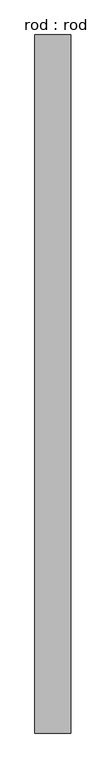
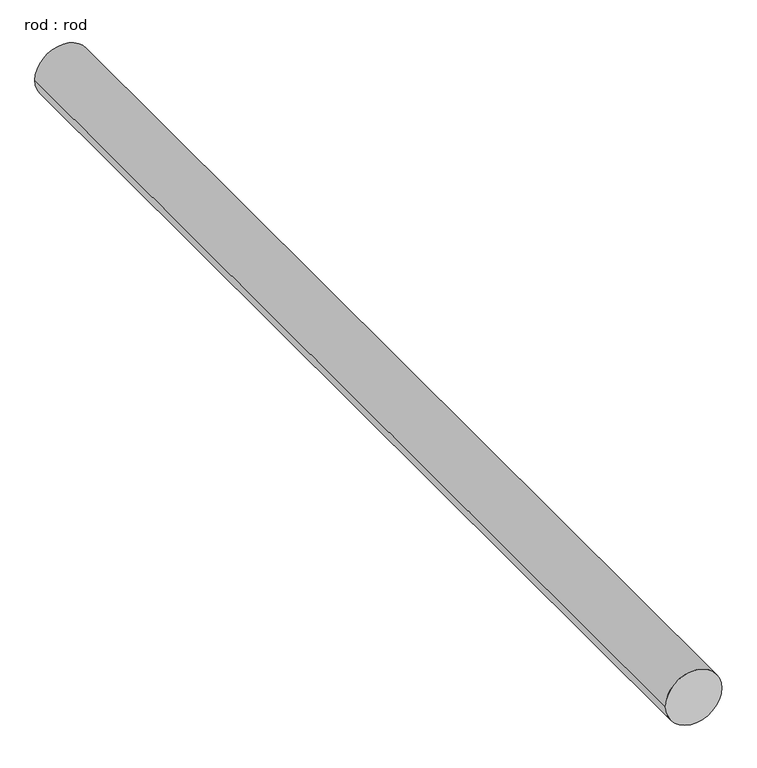
"""IFC4 building model written with IfcOpenShell, lengths in millimetres: proxy geometry, rod : rod."""

from ifc_helpers import new_model, si_unit, point, frame, frame_2d, origin, place, context, project, spatial, circle_curve, trimmed, segment, composite_curve, outline, extrude, source, transform, mapped, element, save


def rod_rod_ac49b040(model_context):
    return source(origin(), model_context, "Body", "SweptSolid", [
        extrude(outline(composite_curve([segment(trimmed(circle_curve(frame_2d((0.0108462, 0.0)), 200.0), [point((0.0108462, 200.0))], [point((0.0108462, -200.0))], False, "CARTESIAN"), True, "CONTINUOUS"), segment(trimmed(circle_curve(frame_2d((0.0108462, 0.0)), 200.0), [point((0.0108462, -200.0))], [point((0.0108462, 200.0))], False, "CARTESIAN"), True, "CONTINUOUS")], self_intersect=False)), frame((0.0, 207.8192318, 0.0), z_axis=(0.0, 1.0, 0.0), x_axis=(0.0, 0.0, 1.0)), (0.0, 0.0, 1.0), 7769.8187671),
    ])


if __name__ == "__main__":
    model = new_model("IFC4")
    model_context = context("Model", 3, world=origin())
    ifc_project = project(units=[si_unit("LENGTHUNIT", "METRE", prefix="MILLI")], contexts=[model_context])
    site = spatial("IfcSite", under=ifc_project)
    building = spatial("IfcBuilding", under=site)
    placement = place(None, origin())
    rod_rod_shape = rod_rod_ac49b040(model_context)
    element("IfcBuildingElementProxy", 1, Name="rod : rod", ObjectType="rod : rod", at=placement, inside=building, context=model_context, shape_type="MappedRepresentation", body=[
        mapped(rod_rod_shape, transform((0.0, 0.0, 0.0), x_axis=(1.0, 0.0, 0.0), y_axis=(0.0, 1.0, 0.0), z_axis=(0.0, 0.0, 1.0))),
    ])
    save(model, "model.ifc")

# Revit data of these elements
# Type "rod : rod"
#   Default Elevation = 0
